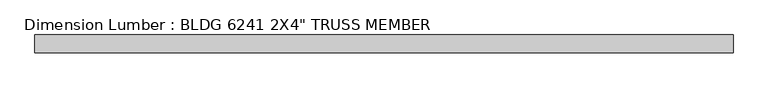
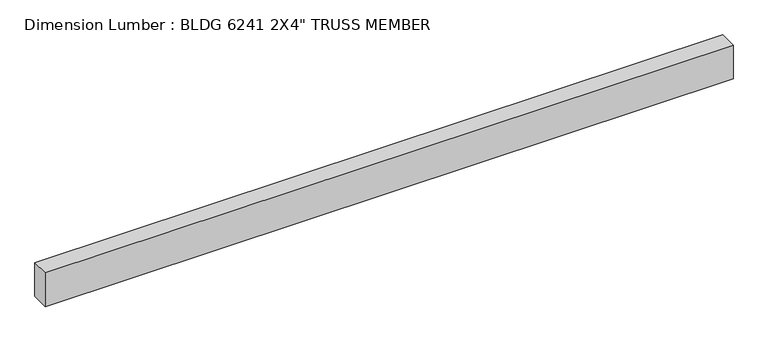
"""IFC4 building model written with IfcOpenShell, lengths in millimetres: beam geometry."""

from ifc_helpers import new_model, si_unit, frame, origin, place, context, project, spatial, polyline, outline, extrude, source, transform, mapped, element, save


def beam_1eeaf63e(model_context):
    return source(origin(), model_context, "Body", "SweptSolid", [
        extrude(outline(polyline([(955.675, 25.4), (955.675, -25.4), (-1006.4749994, -25.4), (-1006.4749994, 25.4), (955.675, 25.4)])), frame((0.0, 0.0, -50.8), z_axis=(0.0, 0.0, 1.0), x_axis=(1.0, 0.0, 0.0)), (0.0, 0.0, 1.0), 101.6),
    ])


if __name__ == "__main__":
    model = new_model("IFC4")
    model_context = context("Model", 3, world=origin())
    ifc_project = project(units=[si_unit("LENGTHUNIT", "METRE", prefix="MILLI")], contexts=[model_context])
    site = spatial("IfcSite", under=ifc_project)
    building = spatial("IfcBuilding", under=site)
    placement = place(None, origin())
    beam_shape = beam_1eeaf63e(model_context)
    element("IfcBeam", 1, ObjectType="Dimension Lumber : BLDG 6241 2X4\" TRUSS MEMBER", at=placement, inside=building, context=model_context, shape_type="MappedRepresentation", body=[
        mapped(beam_shape, transform((0.0, 0.0, 0.0), x_axis=(1.0, 0.0, 0.0), y_axis=(0.0, 1.0, 0.0), z_axis=(0.0, 0.0, 1.0))),
    ])
    save(model, "model.ifc")

# Revit data of these elements
# Type "Dimension Lumber : BLDG 6241 2X4\" TRUSS MEMBER"
#   Assembly Code = "B10"
#   A = 0.273472 SF
#   Length [instance default] = 5' - 0"
#   b = 0' - 2"
#   d = 0' - 4"
#   Structural Material [instance default] = Softwood, Lumber
# Element 1 (IfcBeam, "Dimension Lumber : BLDG 6241 2X4\" TRUSS MEMBER")
#   Materials on its faces: "Softwood, Lumber"
# Materials
#   "Softwood, Lumber": class "Wood", colour RGB 223 192 134, transparency 0, Description = "Pinus Echinata", Cost = 0
